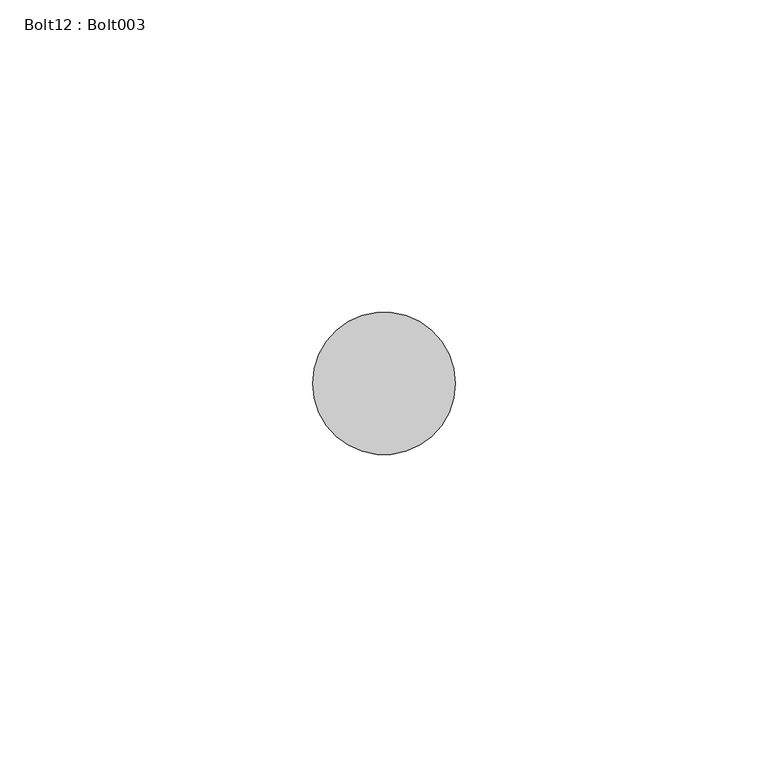
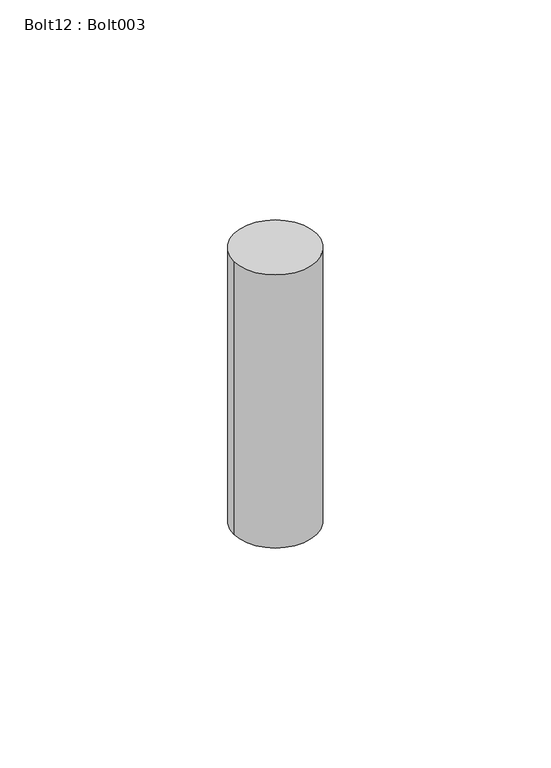
"""IFC4 building model written with IfcOpenShell, lengths in millimetres: proxy geometry, Bolt12 : Bolt003."""

from ifc_helpers import new_model, si_unit, point, frame, frame_2d, origin, place, context, project, spatial, circle_curve, trimmed, segment, composite_curve, outline, extrude, source, transform, mapped, element, save


def bolt12_bolt003_c7632ded(model_context):
    return source(origin(), model_context, "Body", "SweptSolid", [
        extrude(outline(composite_curve([segment(trimmed(circle_curve(frame_2d((5062.3346014, 1998.1882072)), 11.4045168), [point((5073.7391183, 1998.1882072))], [point((5050.9300846, 1998.1882072))], False, "CARTESIAN"), True, "CONTINUOUS"), segment(trimmed(circle_curve(frame_2d((5062.3346014, 1998.1882072)), 11.4045168), [point((5050.9300846, 1998.1882072))], [point((5073.7391183, 1998.1882072))], False, "CARTESIAN"), True, "CONTINUOUS")], self_intersect=False)), frame((0.0, 0.0, 36645.5959962), z_axis=(0.0, 0.0, 1.0), x_axis=(1.0, 0.0, 0.0)), (0.0, 0.0, 1.0), 79.375),
    ])


if __name__ == "__main__":
    model = new_model("IFC4")
    model_context = context("Model", 3, world=origin())
    ifc_project = project(units=[si_unit("LENGTHUNIT", "METRE", prefix="MILLI")], contexts=[model_context])
    site = spatial("IfcSite", under=ifc_project)
    building = spatial("IfcBuilding", under=site)
    placement = place(None, origin())
    bolt12_bolt003_shape = bolt12_bolt003_c7632ded(model_context)
    element("IfcBuildingElementProxy", 1, Name="Bolt12 : Bolt003", ObjectType="Bolt12 : Bolt003", at=placement, inside=building, context=model_context, shape_type="MappedRepresentation", body=[
        mapped(bolt12_bolt003_shape, transform((0.0, 0.0, 0.0), x_axis=(1.0, 0.0, 0.0), y_axis=(0.0, 1.0, 0.0), z_axis=(0.0, 0.0, 1.0))),
    ])
    save(model, "model.ifc")

# Revit data of these elements
# Type "Bolt12 : Bolt003"
#   NameOverride = "Bolt003"
# Element 1 (IfcBuildingElementProxy, "Bolt12 : Bolt003")
#   Materials on its faces: "TUBE STEEL STRINGER WELDED TO ANCHORED STEEL PLATE - SEE STRUCT DWGS"
# Materials
#   "TUBE STEEL STRINGER WELDED TO ANCHORED STEEL PLATE - SEE STRUCT DWGS": class "Unassigned", colour RGB 128 128 128, transparency 0, Cost = 0
